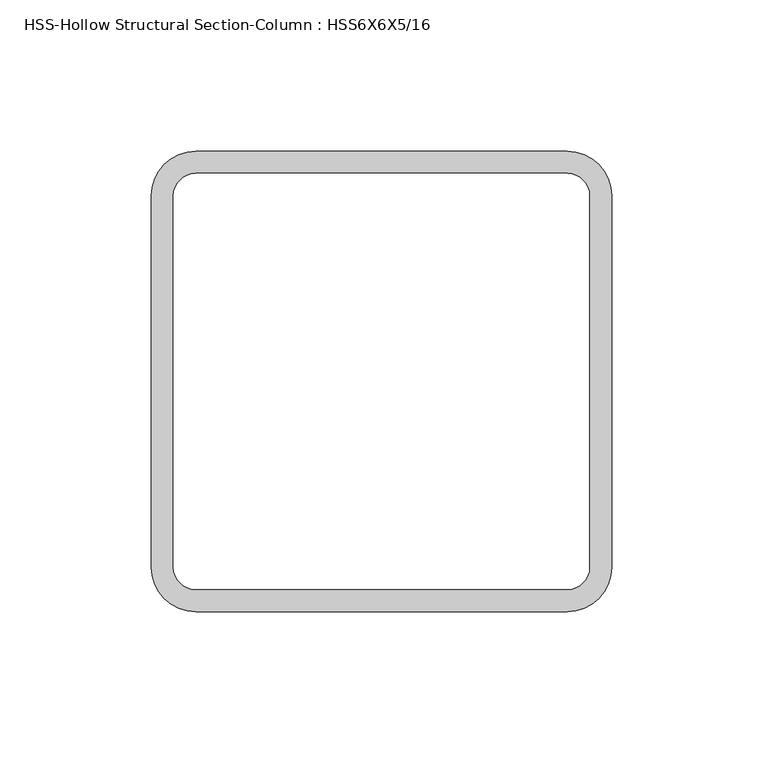
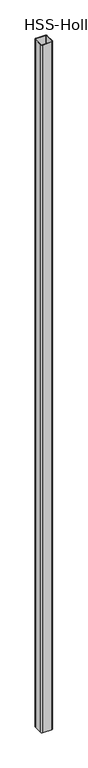
"""IFC4 building model written with IfcOpenShell, lengths in millimetres: column geometry, HSS-Hollow Structural Section-Column : HSS6X6X5/16."""

from ifc_helpers import new_model, si_unit, point, frame, frame_2d, origin, place, context, project, spatial, polyline, circle_curve, trimmed, segment, composite_curve, outline, extrude, source, transform, mapped, element, save


def hss_hollow_structural_section_column_hss6x6x5_16_beb4ea93(model_context):
    return source(origin(), model_context, "Body", "SweptSolid", [
        extrude(outline(composite_curve([segment(trimmed(circle_curve(frame_2d((61.4172, 61.4172)), 14.7828), [point((61.4172, 76.2))], [point((76.2, 61.4172))], False, "CARTESIAN"), True, "CONTINUOUS"), segment(polyline([(76.2, 61.4172), (76.2, -61.4172)]), True, "CONTINUOUS"), segment(trimmed(circle_curve(frame_2d((61.4172, -61.4172)), 14.7828), [point((76.2, -61.4172))], [point((61.4172, -76.2))], False, "CARTESIAN"), True, "CONTINUOUS"), segment(polyline([(61.4172, -76.2), (-61.4172, -76.2)]), True, "CONTINUOUS"), segment(trimmed(circle_curve(frame_2d((-61.4172, -61.4172)), 14.7828), [point((-61.4172, -76.2))], [point((-76.2, -61.4172))], False, "CARTESIAN"), True, "CONTINUOUS"), segment(polyline([(-76.2, -61.4172), (-76.2, 61.4172)]), True, "CONTINUOUS"), segment(trimmed(circle_curve(frame_2d((-61.4172, 61.4172)), 14.7828), [point((-76.2, 61.4172))], [point((-61.4172, 76.2))], False, "CARTESIAN"), True, "CONTINUOUS"), segment(polyline([(-61.4172, 76.2), (61.4172, 76.2)]), True, "CONTINUOUS")], self_intersect=False), holes=[composite_curve([segment(polyline([(61.4172, 68.8086), (-61.4172, 68.8086)]), True, "CONTINUOUS"), segment(trimmed(circle_curve(frame_2d((-61.4172, 61.4172)), 7.3914), [point((-61.4172, 68.8086))], [point((-68.8086, 61.4172))], True, "CARTESIAN"), True, "CONTINUOUS"), segment(polyline([(-68.8086, 61.4172), (-68.8086, -61.4172)]), True, "CONTINUOUS"), segment(trimmed(circle_curve(frame_2d((-61.4172, -61.4172)), 7.3914), [point((-68.8086, -61.4172))], [point((-61.4172, -68.8086))], True, "CARTESIAN"), True, "CONTINUOUS"), segment(polyline([(-61.4172, -68.8086), (61.4172, -68.8086)]), True, "CONTINUOUS"), segment(trimmed(circle_curve(frame_2d((61.4172, -61.4172)), 7.3914), [point((61.4172, -68.8086))], [point((68.8086, -61.4172))], True, "CARTESIAN"), True, "CONTINUOUS"), segment(polyline([(68.8086, -61.4172), (68.8086, 61.4172)]), True, "CONTINUOUS"), segment(trimmed(circle_curve(frame_2d((61.4172, 61.4172)), 7.3914), [point((68.8086, 61.4172))], [point((61.4172, 68.8086))], True, "CARTESIAN"), True, "CONTINUOUS")], self_intersect=False)]), frame((0.0, 0.0, 12566.65), z_axis=(0.0, 0.0, 1.0), x_axis=(1.0, 0.0, 0.0)), (0.0, 0.0, 1.0), 9531.35),
    ])


if __name__ == "__main__":
    model = new_model("IFC4")
    model_context = context("Model", 3, world=origin())
    ifc_project = project(units=[si_unit("LENGTHUNIT", "METRE", prefix="MILLI")], contexts=[model_context])
    site = spatial("IfcSite", under=ifc_project)
    building = spatial("IfcBuilding", under=site)
    placement = place(None, origin())
    hss_hollow_structural_section_column_hss6x6x5_16_shape = hss_hollow_structural_section_column_hss6x6x5_16_beb4ea93(model_context)
    element("IfcColumn", 1, ObjectType="HSS-Hollow Structural Section-Column : HSS6X6X5/16", at=placement, inside=building, context=model_context, shape_type="MappedRepresentation", body=[
        mapped(hss_hollow_structural_section_column_hss6x6x5_16_shape, transform((0.0, 0.0, 0.0), x_axis=(1.0, 0.0, 0.0), y_axis=(0.0, 1.0, 0.0), z_axis=(0.0, 0.0, 1.0))),
    ])
    save(model, "model.ifc")

# Revit data of these elements
# Type "HSS-Hollow Structural Section-Column : HSS6X6X5/16"
#   Assembly Code = "B10"
#   Shape = "Square"
#   W = 23.3
#   Ht = 0' - 6"
#   b = 0' - 6"
#   kr = 0' - 0.582"
#   t = 0' - 0.291"
#   A = 0.0446528 SF
#   Structural Material [instance default] = Steel ASTM A500, Grade B, Rectangular and Square
# Element 1 (IfcColumn, "HSS-Hollow Structural Section-Column : HSS6X6X5/16")
#   Materials on its faces: "Steel ASTM A500, Grade B, Rectangular and Square"
# Materials
#   "Steel ASTM A500, Grade B, Rectangular and Square": class "Metal", colour RGB 199 199 199, transparency 0, Description = "Carbon steel", Cost = 0
